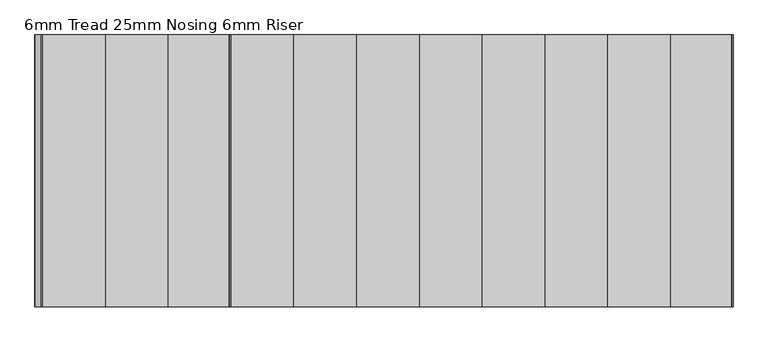
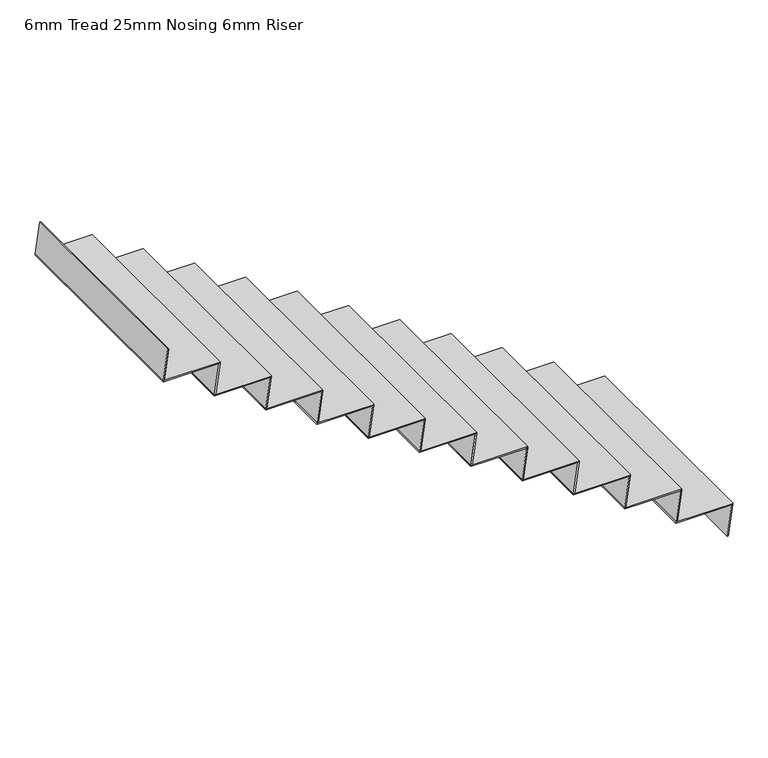
"""IFC4 building model written with IfcOpenShell, lengths in millimetres: stair flight geometry, 6mm Tread 25mm Nosing 6mm Riser."""

from ifc_helpers import new_model, si_unit, frame, origin, place, context, project, spatial, polyline, outline, extrude, source, transform, mapped, element, save


def stair_flight_6mm_tread_25mm_nosing_6mm_riser_7ebcc734(model_context):
    return source(origin(), model_context, "Body", "SweptSolid", [
        extrude(outline(polyline([(14352.9411765, 16350.0), (14352.9411765, 16043.9400908), (14346.9411765, 16043.0900908), (14346.9411765, 16349.15), (14352.9411765, 16350.0)])), frame((0.0, 12030.4345331, 0.0), z_axis=(0.0, 1.0, 0.0), x_axis=(0.0, 0.0, 1.0)), (0.0, 0.0, 1.0), 1190.0),
        extrude(outline(polyline([(14346.9411765, 16349.15), (14346.9411765, 16343.0900908), (14176.4705882, 16318.9400908), (14176.4705882, 16325.0), (14346.9411765, 16349.15)])), frame((0.0, 12030.4345331, 0.0), z_axis=(0.0, 1.0, 0.0), x_axis=(0.0, 0.0, 1.0)), (0.0, 0.0, 1.0), 1190.0),
        extrude(outline(polyline([(14523.4117647, 16074.15), (14523.4117647, 16068.0900908), (14352.9411765, 16043.9400908), (14352.9411765, 16050.0), (14523.4117647, 16074.15)])), frame((0.0, 12030.4345331, 0.0), z_axis=(0.0, 1.0, 0.0), x_axis=(0.0, 0.0, 1.0)), (0.0, 0.0, 1.0), 1190.0),
        extrude(outline(polyline([(14529.4117647, 16075.0), (14529.4117647, 15768.9400908), (14523.4117647, 15768.0900908), (14523.4117647, 16074.15), (14529.4117647, 16075.0)])), frame((0.0, 12030.4345331, 0.0), z_axis=(0.0, 1.0, 0.0), x_axis=(0.0, 0.0, 1.0)), (0.0, 0.0, 1.0), 1190.0),
        extrude(outline(polyline([(14699.8823529, 15799.15), (14699.8823529, 15793.0900908), (14529.4117647, 15768.9400908), (14529.4117647, 15775.0), (14699.8823529, 15799.15)])), frame((0.0, 12030.4345331, 0.0), z_axis=(0.0, 1.0, 0.0), x_axis=(0.0, 0.0, 1.0)), (0.0, 0.0, 1.0), 1190.0),
        extrude(outline(polyline([(14705.8823529, 15800.0), (14705.8823529, 15493.9400908), (14699.8823529, 15493.0900908), (14699.8823529, 15799.15), (14705.8823529, 15800.0)])), frame((0.0, 12030.4345331, 0.0), z_axis=(0.0, 1.0, 0.0), x_axis=(0.0, 0.0, 1.0)), (0.0, 0.0, 1.0), 1190.0),
        extrude(outline(polyline([(14876.3529412, 15524.15), (14876.3529412, 15518.0900908), (14705.8823529, 15493.9400908), (14705.8823529, 15500.0), (14876.3529412, 15524.15)])), frame((0.0, 12030.4345331, 0.0), z_axis=(0.0, 1.0, 0.0), x_axis=(0.0, 0.0, 1.0)), (0.0, 0.0, 1.0), 1190.0),
        extrude(outline(polyline([(14882.3529412, 15525.0), (14882.3529412, 15218.9400908), (14876.3529412, 15218.0900908), (14876.3529412, 15524.15), (14882.3529412, 15525.0)])), frame((0.0, 12030.4345331, 0.0), z_axis=(0.0, 1.0, 0.0), x_axis=(0.0, 0.0, 1.0)), (0.0, 0.0, 1.0), 1190.0),
        extrude(outline(polyline([(15052.8235294, 15249.15), (15052.8235294, 15243.0900908), (14882.3529412, 15218.9400908), (14882.3529412, 15225.0), (15052.8235294, 15249.15)])), frame((0.0, 12030.4345331, 0.0), z_axis=(0.0, 1.0, 0.0), x_axis=(0.0, 0.0, 1.0)), (0.0, 0.0, 1.0), 1190.0),
        extrude(outline(polyline([(15058.8235294, 15250.0), (15058.8235294, 14943.9400908), (15052.8235294, 14943.0900908), (15052.8235294, 15249.15), (15058.8235294, 15250.0)])), frame((0.0, 12030.4345331, 0.0), z_axis=(0.0, 1.0, 0.0), x_axis=(0.0, 0.0, 1.0)), (0.0, 0.0, 1.0), 1190.0),
        extrude(outline(polyline([(15229.2941176, 14974.15), (15229.2941176, 14968.0900908), (15058.8235294, 14943.9400908), (15058.8235294, 14950.0), (15229.2941176, 14974.15)])), frame((0.0, 12030.4345331, 0.0), z_axis=(0.0, 1.0, 0.0), x_axis=(0.0, 0.0, 1.0)), (0.0, 0.0, 1.0), 1190.0),
        extrude(outline(polyline([(15235.2941176, 14975.0), (15235.2941176, 14668.9400908), (15229.2941176, 14668.0900908), (15229.2941176, 14974.15), (15235.2941176, 14975.0)])), frame((0.0, 12030.4345331, 0.0), z_axis=(0.0, 1.0, 0.0), x_axis=(0.0, 0.0, 1.0)), (0.0, 0.0, 1.0), 1190.0),
        extrude(outline(polyline([(15405.7647059, 14699.15), (15405.7647059, 14693.0900908), (15235.2941176, 14668.9400908), (15235.2941176, 14675.0), (15405.7647059, 14699.15)])), frame((0.0, 12030.4345331, 0.0), z_axis=(0.0, 1.0, 0.0), x_axis=(0.0, 0.0, 1.0)), (0.0, 0.0, 1.0), 1190.0),
        extrude(outline(polyline([(15411.7647059, 14700.0), (15411.7647059, 14393.9400908), (15405.7647059, 14393.0900908), (15405.7647059, 14699.15), (15411.7647059, 14700.0)])), frame((0.0, 12030.4345331, 0.0), z_axis=(0.0, 1.0, 0.0), x_axis=(0.0, 0.0, 1.0)), (0.0, 0.0, 1.0), 1190.0),
        extrude(outline(polyline([(15582.2352941, 14424.15), (15582.2352941, 14418.0900908), (15411.7647059, 14393.9400908), (15411.7647059, 14400.0), (15582.2352941, 14424.15)])), frame((0.0, 12030.4345331, 0.0), z_axis=(0.0, 1.0, 0.0), x_axis=(0.0, 0.0, 1.0)), (0.0, 0.0, 1.0), 1190.0),
        extrude(outline(polyline([(15588.2352941, 14425.0), (15588.2352941, 14118.9400908), (15582.2352941, 14118.0900908), (15582.2352941, 14424.15), (15588.2352941, 14425.0)])), frame((0.0, 12030.4345331, 0.0), z_axis=(0.0, 1.0, 0.0), x_axis=(0.0, 0.0, 1.0)), (0.0, 0.0, 1.0), 1190.0),
        extrude(outline(polyline([(15758.7058824, 14149.15), (15758.7058824, 14143.0900908), (15588.2352941, 14118.9400908), (15588.2352941, 14125.0), (15758.7058824, 14149.15)])), frame((0.0, 12030.4345331, 0.0), z_axis=(0.0, 1.0, 0.0), x_axis=(0.0, 0.0, 1.0)), (0.0, 0.0, 1.0), 1190.0),
        extrude(outline(polyline([(15764.7058824, 14150.0), (15764.7058824, 13843.9400908), (15758.7058824, 13843.0900908), (15758.7058824, 14149.15), (15764.7058824, 14150.0)])), frame((0.0, 12030.4345331, 0.0), z_axis=(0.0, 1.0, 0.0), x_axis=(0.0, 0.0, 1.0)), (0.0, 0.0, 1.0), 1190.0),
        extrude(outline(polyline([(15935.1764706, 13874.15), (15935.1764706, 13868.0900908), (15764.7058824, 13843.9400908), (15764.7058824, 13850.0), (15935.1764706, 13874.15)])), frame((0.0, 12030.4345331, 0.0), z_axis=(0.0, 1.0, 0.0), x_axis=(0.0, 0.0, 1.0)), (0.0, 0.0, 1.0), 1190.0),
        extrude(outline(polyline([(15941.1764706, 13875.0), (15941.1764706, 13568.9400908), (15935.1764706, 13568.0900908), (15935.1764706, 13874.15), (15941.1764706, 13875.0)])), frame((0.0, 12030.4345331, 0.0), z_axis=(0.0, 1.0, 0.0), x_axis=(0.0, 0.0, 1.0)), (0.0, 0.0, 1.0), 1190.0),
        extrude(outline(polyline([(16111.6470588, 13599.15), (16111.6470588, 13593.0900908), (15941.1764706, 13568.9400908), (15941.1764706, 13575.0), (16111.6470588, 13599.15)])), frame((0.0, 12030.4345331, 0.0), z_axis=(0.0, 1.0, 0.0), x_axis=(0.0, 0.0, 1.0)), (0.0, 0.0, 1.0), 1190.0),
        extrude(outline(polyline([(16288.1176471, 13324.15), (16288.1176471, 13318.0900908), (16117.6470588, 13293.9400908), (16117.6470588, 13300.0), (16288.1176471, 13324.15)])), frame((0.0, 12030.4345331, 0.0), z_axis=(0.0, 1.0, 0.0), x_axis=(0.0, 0.0, 1.0)), (0.0, 0.0, 1.0), 1190.0),
        extrude(outline(polyline([(16117.6470588, 13600.0), (16117.6470588, 13293.9400908), (16111.6470588, 13293.0900908), (16111.6470588, 13599.15), (16117.6470588, 13600.0)])), frame((0.0, 12030.4345331, 0.0), z_axis=(0.0, 1.0, 0.0), x_axis=(0.0, 0.0, 1.0)), (0.0, 0.0, 1.0), 1190.0),
    ])


if __name__ == "__main__":
    model = new_model("IFC4")
    model_context = context("Model", 3, world=origin())
    ifc_project = project(units=[si_unit("LENGTHUNIT", "METRE", prefix="MILLI")], contexts=[model_context])
    site = spatial("IfcSite", under=ifc_project)
    building = spatial("IfcBuilding", under=site)
    placement = place(None, origin())
    stair_flight_6mm_tread_25mm_nosing_6mm_riser_shape = stair_flight_6mm_tread_25mm_nosing_6mm_riser_7ebcc734(model_context)
    element("IfcStairFlight", 1, ObjectType="6mm Tread 25mm Nosing 6mm Riser", at=placement, inside=building, context=model_context, shape_type="MappedRepresentation", body=[
        mapped(stair_flight_6mm_tread_25mm_nosing_6mm_riser_shape, transform((0.0, 0.0, 0.0), x_axis=(1.0, 0.0, 0.0), y_axis=(0.0, 1.0, 0.0), z_axis=(0.0, 0.0, 1.0))),
    ])
    save(model, "model.ifc")

# Revit data of these elements
# Element 1 (IfcStairFlight, "6mm Tread 25mm Nosing 6mm Riser")
#   Materials on its faces: "Steel, Paint Finish, Dark Gray"
# Materials
#   "Steel, Paint Finish, Dark Gray": class "Metal", colour RGB 89 89 89, transparency 0, Description = "Steel, paint finish, dark gray, glossy", Cost = 0
